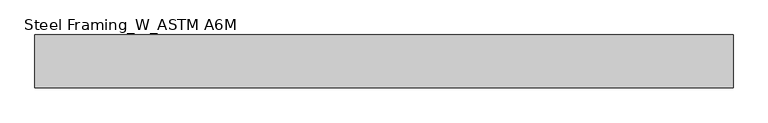
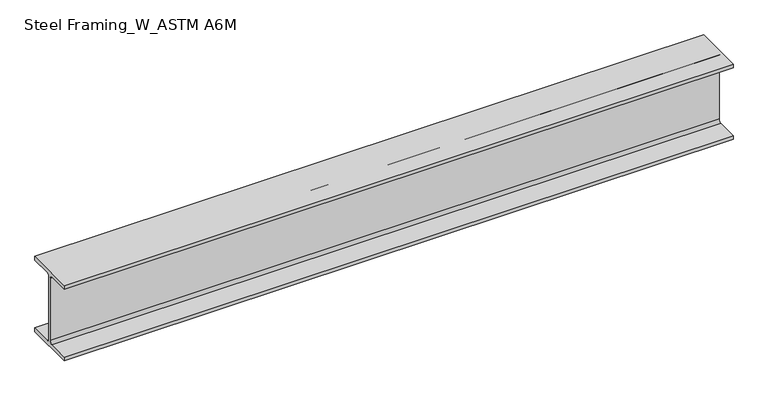
"""IFC4 building model written with IfcOpenShell, lengths in millimetres: beam geometry, Steel Framing_W_ASTM A6M : H_SB_AR_S02_W200x31.3_B6."""

import ifcopenshell
import ifcopenshell.guid

model = None  # the IFC model being written
_history = None  # IfcOwnerHistory: only IFC2X3 demands one
_inside = {}  # id of a spatial element -> (the spatial element, [elements in it])
_under = {}  # id of a project, library or spatial element -> (it, [spatial elements below it])
_declared = {}  # id of a project -> (the project, [libraries it declares])
_typed = {}  # id of a type object -> (the type object, [elements of that type])
_made_of = {}  # id of a material, layer set ... -> (it, [elements and type objects made of it])


def new_model(schema):
    """Start an empty IFC model of exactly this schema.

    Asked for "IFC4X3", IfcOpenShell would pick the latest addendum, in which some entities
    have other attributes; the version numbers below select the first issue.
    IFC2X3 requires an IfcOwnerHistory on every rooted entity: one is made here for all.
    """
    global model, _history
    if schema == "IFC4X3":
        model = ifcopenshell.file(schema_version=(4, 3, 0, 0))
    else:
        model = ifcopenshell.file(schema=schema)
    _inside.clear()
    _under.clear()
    _declared.clear()
    _typed.clear()
    _made_of.clear()
    _history = None
    if model.schema == "IFC2X3":
        org = make("IfcOrganization", Name="unknown")
        user = make(
            "IfcPersonAndOrganization",
            ThePerson=make("IfcPerson", FamilyName="unknown"),
            TheOrganization=org,
        )
        app = make(
            "IfcApplication",
            ApplicationDeveloper=org,
            Version="unknown",
            ApplicationFullName="unknown",
            ApplicationIdentifier="unknown",
        )
        _history = make(
            "IfcOwnerHistory",
            OwningUser=user,
            OwningApplication=app,
            ChangeAction="ADDED",
            CreationDate=0,
        )
    return model


def make(cls, **values):
    """One entity of the class cls with the attributes given. An attribute that is None is left unset."""
    return model.create_entity(
        cls, **{name: value for name, value in values.items() if value is not None}
    )


def rooted(cls, **values):
    """An entity with a GlobalId (a new one), such as an element, a storey or a relation."""
    return make(cls, GlobalId=ifcopenshell.guid.new(), OwnerHistory=_history, **values)


def si_unit(unit_type, name, prefix=None):
    """IfcSIUnit, for example si_unit("LENGTHUNIT", "METRE", prefix="MILLI")."""
    return make("IfcSIUnit", UnitType=unit_type, Prefix=prefix, Name=name)


def assignment(units):
    """IfcUnitAssignment: the units of a project."""
    return None if units is None else make("IfcUnitAssignment", Units=units)


def point(xyz):
    """IfcCartesianPoint."""
    return None if xyz is None else make("IfcCartesianPoint", Coordinates=xyz)


def direction(xyz):
    """IfcDirection."""
    return None if xyz is None else make("IfcDirection", DirectionRatios=xyz)


def frame(location, z_axis=None, x_axis=None):
    """IfcAxis2Placement3D, a coordinate frame: its origin and axes. An axis left out is left unset."""
    return make(
        "IfcAxis2Placement3D",
        Location=point(location),
        Axis=direction(z_axis),
        RefDirection=direction(x_axis),
    )


def frame_2d(location, x_axis=None):
    """IfcAxis2Placement2D, a coordinate frame in the plane: its origin and x axis."""
    return make(
        "IfcAxis2Placement2D", Location=point(location), RefDirection=direction(x_axis)
    )


def origin():
    """The frame at (0, 0, 0) with its axes left unset."""
    return frame((0.0, 0.0, 0.0))


def place(relative_to, where):
    """IfcLocalPlacement: puts the frame where relative to a parent placement (None: the world)."""
    return make(
        "IfcLocalPlacement", PlacementRelTo=relative_to, RelativePlacement=where
    )


def context(
    kind, dimensions, precision=None, world=None, true_north=None, identifier=None
):
    """IfcGeometricRepresentationContext, for example the 3D "Model" context."""
    return make(
        "IfcGeometricRepresentationContext",
        ContextIdentifier=identifier,
        ContextType=kind,
        CoordinateSpaceDimension=dimensions,
        Precision=precision,
        WorldCoordinateSystem=world,
        TrueNorth=true_north,
    )


def project(units=None, contexts=None):
    """IfcProject with its units and contexts."""
    return rooted(
        "IfcProject",
        Name="project",
        RepresentationContexts=contexts,
        UnitsInContext=assignment(units),
    )


def spatial(cls, under=None, at=None, **own):
    """A site, building, storey or space (cls), placed at a placement, below another one or the project."""
    s = rooted(cls, ObjectPlacement=at, **own)
    if under is not None:
        _under.setdefault(under.id(), (under, []))[1].append(s)
    return s


def polyline(points):
    """IfcPolyline through the points."""
    return make("IfcPolyline", Points=[point(p) for p in points])


def circle_curve(where, radius):
    """IfcCircle in the frame where."""
    return make("IfcCircle", Position=where, Radius=radius)


def trimmed(basis, trim1, trim2, sense, master):
    """IfcTrimmedCurve: the piece of a basis curve between two trims."""
    return make(
        "IfcTrimmedCurve",
        BasisCurve=basis,
        Trim1=trim1,
        Trim2=trim2,
        SenseAgreement=sense,
        MasterRepresentation=master,
    )


def segment(curve, same_sense, transition):
    """IfcCompositeCurveSegment."""
    return make(
        "IfcCompositeCurveSegment",
        Transition=transition,
        SameSense=same_sense,
        ParentCurve=curve,
    )


def composite_curve(segments, self_intersect=None):
    """IfcCompositeCurve: segments joined end to end."""
    return make("IfcCompositeCurve", Segments=segments, SelfIntersect=self_intersect)


def outline(outer, holes=None, kind="AREA"):
    """IfcArbitraryClosedProfileDef: a profile drawn as a closed curve; with holes, ...WithVoids."""
    if holes is None:
        return make("IfcArbitraryClosedProfileDef", ProfileType=kind, OuterCurve=outer)
    return make(
        "IfcArbitraryProfileDefWithVoids",
        ProfileType=kind,
        OuterCurve=outer,
        InnerCurves=holes,
    )


def extrude(swept, where, along, depth):
    """IfcExtrudedAreaSolid: the profile swept, set in the frame where, extruded along a direction by depth."""
    return make(
        "IfcExtrudedAreaSolid",
        SweptArea=swept,
        Position=where,
        ExtrudedDirection=direction(along),
        Depth=depth,
    )


def shape(context_of_items, identifier, shape_type, items):
    """IfcShapeRepresentation: the items that make up one representation, for example the "Body"."""
    return make(
        "IfcShapeRepresentation",
        ContextOfItems=context_of_items,
        RepresentationIdentifier=identifier,
        RepresentationType=shape_type,
        Items=items,
    )


def source(mapping_origin, context_of_items, identifier, shape_type, items):
    """IfcRepresentationMap: a shape defined once, which mapped items show again and again."""
    return make(
        "IfcRepresentationMap",
        MappingOrigin=mapping_origin,
        MappedRepresentation=shape(context_of_items, identifier, shape_type, items),
    )


def transform(
    local_origin,
    x_axis=None,
    y_axis=None,
    z_axis=None,
    scale=None,
    scale2=None,
    scale3=None,
    uniform=True,
):
    """IfcCartesianTransformationOperator3D, or its non-uniform kind. x_axis, y_axis, z_axis: its Axis1, 2, 3."""
    if uniform:
        return make(
            "IfcCartesianTransformationOperator3D",
            Axis1=direction(x_axis),
            Axis2=direction(y_axis),
            LocalOrigin=point(local_origin),
            Scale=scale,
            Axis3=direction(z_axis),
        )
    return make(
        "IfcCartesianTransformationOperator3DnonUniform",
        Axis1=direction(x_axis),
        Axis2=direction(y_axis),
        LocalOrigin=point(local_origin),
        Scale=scale,
        Axis3=direction(z_axis),
        Scale2=scale2,
        Scale3=scale3,
    )


def mapped(mapping_source, mapping_target):
    """IfcMappedItem: shows the shape of a source again, moved by a transform."""
    return make(
        "IfcMappedItem", MappingSource=mapping_source, MappingTarget=mapping_target
    )


def made_of(thing, what):
    """Note that an element or type object is made of a material, layer set ...; save() writes the relation."""
    if what is not None:
        _made_of.setdefault(what.id(), (what, []))[1].append(thing)
    return thing


def element(
    cls,
    number,
    at=None,
    inside=None,
    cuts=None,
    type_object=None,
    material=None,
    context=None,
    identifier="Body",
    shape_type=None,
    held_by="IfcProductDefinitionShape",
    body=None,
    shapes=None,
    **own,
):
    """One element of the class cls, such as IfcWall. Its Tag is "e" and its number.

    at: its placement. inside: the storey or other place that contains it. cuts: it is an
    opening in that element (IfcRelVoidsElement). A single representation is given by context,
    identifier, shape_type and body (its items); several are given by shapes. held_by: the class
    of the entity that holds the representations. save() writes the other relations.
    """
    e = rooted(cls, Tag="e%d" % number, ObjectPlacement=at, **own)
    if body is not None:
        shapes = [shape(context, identifier, shape_type, body)]
    if shapes is not None:
        e.Representation = make(held_by, Representations=shapes)
    if inside is not None:
        _inside.setdefault(inside.id(), (inside, []))[1].append(e)
    if cuts is not None:
        rooted(
            "IfcRelVoidsElement", RelatingBuildingElement=cuts, RelatedOpeningElement=e
        )
    if type_object is not None:
        _typed.setdefault(type_object.id(), (type_object, []))[1].append(e)
    return made_of(e, material)


def aggregate(whole, parts):
    """IfcRelAggregates: a whole, such as a stair, and the parts it consists of."""
    return rooted("IfcRelAggregates", RelatingObject=whole, RelatedObjects=parts)


def save(model, path):
    """Write the relations noted so far, then the file.

    IfcRelAggregates (storeys below a building ...), IfcRelContainedInSpatialStructure (elements
    in a storey), IfcRelDefinesByType, IfcRelAssociatesMaterial and IfcRelDeclares: one each for
    every whole, place, type object, material and project.
    """
    for whole, parts in _under.values():
        aggregate(whole, parts)
    for where, things in _inside.values():
        rooted(
            "IfcRelContainedInSpatialStructure",
            RelatedElements=things,
            RelatingStructure=where,
        )
    for kind, things in _typed.values():
        rooted("IfcRelDefinesByType", RelatedObjects=things, RelatingType=kind)
    for what, things in _made_of.values():
        rooted("IfcRelAssociatesMaterial", RelatedObjects=things, RelatingMaterial=what)
    for by, libraries in _declared.values():
        rooted("IfcRelDeclares", RelatingContext=by, RelatedDefinitions=libraries)
    model.write(path)


def steel_framing_w_astm_a6m_cb9fb0c6(model_context):
    return source(origin(), model_context, "Body", "SweptSolid", [
        extrude(outline(composite_curve([segment(polyline([(67.0, -94.8), (67.0, -105.0), (-67.0, -105.0), (-67.0, -94.8), (-10.775, -94.8)]), True, "CONTINUOUS"), segment(trimmed(circle_curve(frame_2d((-10.775, -87.2)), 7.6), [point((-10.775, -94.8))], [point((-3.175, -87.2))], True, "CARTESIAN"), True, "CONTINUOUS"), segment(polyline([(-3.175, -87.2), (-3.175, 87.2)]), True, "CONTINUOUS"), segment(trimmed(circle_curve(frame_2d((-10.775, 87.2)), 7.6), [point((-3.175, 87.2))], [point((-10.775, 94.8))], True, "CARTESIAN"), True, "CONTINUOUS"), segment(polyline([(-10.775, 94.8), (-67.0, 94.8), (-67.0, 105.0), (67.0, 105.0), (67.0, 94.8), (10.775, 94.8)]), True, "CONTINUOUS"), segment(trimmed(circle_curve(frame_2d((10.775, 87.2)), 7.6), [point((10.775, 94.8))], [point((3.175, 87.2))], True, "CARTESIAN"), True, "CONTINUOUS"), segment(polyline([(3.175, 87.2), (3.175, -87.2)]), True, "CONTINUOUS"), segment(trimmed(circle_curve(frame_2d((10.775, -87.2)), 7.6), [point((3.175, -87.2))], [point((10.775, -94.8))], True, "CARTESIAN"), True, "CONTINUOUS"), segment(polyline([(10.775, -94.8), (67.0, -94.8)]), True, "CONTINUOUS")], self_intersect=False)), frame((-846.3, 0.0, 0.0), z_axis=(1.0, 0.0, 0.0), x_axis=(0.0, 1.0, 0.0)), (0.0, 0.0, 1.0), 1766.6),
    ])


if __name__ == "__main__":
    model = new_model("IFC4")
    model_context = context("Model", 3, world=origin())
    ifc_project = project(units=[si_unit("LENGTHUNIT", "METRE", prefix="MILLI")], contexts=[model_context])
    site = spatial("IfcSite", under=ifc_project)
    building = spatial("IfcBuilding", under=site)
    placement = place(None, origin())
    steel_framing_w_astm_a6m_shape = steel_framing_w_astm_a6m_cb9fb0c6(model_context)
    element("IfcBeam", 1, ObjectType="Steel Framing_W_ASTM A6M : H_SB_AR_S02_W200x31.3_B6", at=placement, inside=building, context=model_context, shape_type="MappedRepresentation", body=[
        mapped(steel_framing_w_astm_a6m_shape, transform((0.0, 0.0, 0.0), x_axis=(1.0, 0.0, 0.0), y_axis=(0.0, 1.0, 0.0), z_axis=(0.0, 0.0, 1.0))),
    ])
    save(model, "model.ifc")

# Revit data of these elements
# Type "Steel Framing_W_ASTM A6M : H_SB_AR_S02_W200x31.3_B6"
#   Type Mark = "B6"
#   Section Name Key = "W8x21"
#   Width = 13.4 cm
#   Web Thickness = 0.635 cm
#   Web Fillet = 0.76 cm
#   Warping Constant = 40800.0 cm⁶
#   Torsional Moment of Inertia = 11.70 cm⁴
#   Section Area = 39.7 cm²
#   Plastic Modulus weak axis = 93.2 cm³
#   Plastic Modulus strong axis = 334.0 cm³
#   Perimeter = 0.93 m²/m
#   Nominal Weight = 31.30 kgf/m
#   Moment of Inertia weak axis = 407.00 cm⁴
#   Moment of Inertia strong axis = 3130.00 cm⁴
#   Height = 21.0 cm
#   Flange Thickness = 1.02 cm
#   Elastic Modulus weak axis = 60.8 cm³
#   Elastic Modulus strong axis = 298.0 cm³
#   Centroid Vertical = 10.5 cm
#   Centroid Horizontal = 6.7 cm
#   Length [instance default] = 1500 mm
#   Structural Material [instance default] = Steel, 45-345
#   Bolt Spacing = 0
#   Assembly Code = ""
# Element 1 (IfcBeam, "Steel Framing_W_ASTM A6M : H_SB_AR_S02_W200x31.3_B6")
#   Materials on its faces: "Steel, 45-345"
# Materials
#   "Steel, 45-345": class "Metal", colour RGB 189 187 185, transparency 0, Description = "Steel 345 MPa", Cost = 0
